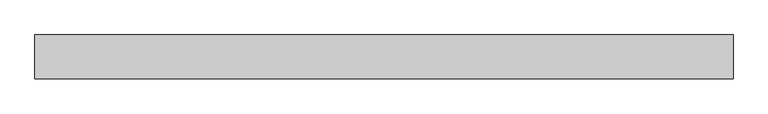
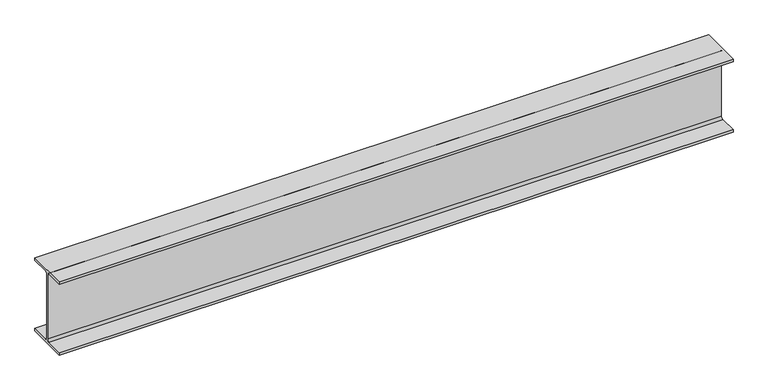
"""IFC4 building model written with IfcOpenShell, lengths in millimetres: beam geometry, Steel Beam_H-KSD3502 : H_SB_ASB_H-250x125x6x9."""

import ifcopenshell
import ifcopenshell.guid

model = None  # the IFC model being written
_history = None  # IfcOwnerHistory: only IFC2X3 demands one
_inside = {}  # id of a spatial element -> (the spatial element, [elements in it])
_under = {}  # id of a project, library or spatial element -> (it, [spatial elements below it])
_declared = {}  # id of a project -> (the project, [libraries it declares])
_typed = {}  # id of a type object -> (the type object, [elements of that type])
_made_of = {}  # id of a material, layer set ... -> (it, [elements and type objects made of it])


def new_model(schema):
    """Start an empty IFC model of exactly this schema.

    Asked for "IFC4X3", IfcOpenShell would pick the latest addendum, in which some entities
    have other attributes; the version numbers below select the first issue.
    IFC2X3 requires an IfcOwnerHistory on every rooted entity: one is made here for all.
    """
    global model, _history
    if schema == "IFC4X3":
        model = ifcopenshell.file(schema_version=(4, 3, 0, 0))
    else:
        model = ifcopenshell.file(schema=schema)
    _inside.clear()
    _under.clear()
    _declared.clear()
    _typed.clear()
    _made_of.clear()
    _history = None
    if model.schema == "IFC2X3":
        org = make("IfcOrganization", Name="unknown")
        user = make(
            "IfcPersonAndOrganization",
            ThePerson=make("IfcPerson", FamilyName="unknown"),
            TheOrganization=org,
        )
        app = make(
            "IfcApplication",
            ApplicationDeveloper=org,
            Version="unknown",
            ApplicationFullName="unknown",
            ApplicationIdentifier="unknown",
        )
        _history = make(
            "IfcOwnerHistory",
            OwningUser=user,
            OwningApplication=app,
            ChangeAction="ADDED",
            CreationDate=0,
        )
    return model


def make(cls, **values):
    """One entity of the class cls with the attributes given. An attribute that is None is left unset."""
    return model.create_entity(
        cls, **{name: value for name, value in values.items() if value is not None}
    )


def rooted(cls, **values):
    """An entity with a GlobalId (a new one), such as an element, a storey or a relation."""
    return make(cls, GlobalId=ifcopenshell.guid.new(), OwnerHistory=_history, **values)


def si_unit(unit_type, name, prefix=None):
    """IfcSIUnit, for example si_unit("LENGTHUNIT", "METRE", prefix="MILLI")."""
    return make("IfcSIUnit", UnitType=unit_type, Prefix=prefix, Name=name)


def assignment(units):
    """IfcUnitAssignment: the units of a project."""
    return None if units is None else make("IfcUnitAssignment", Units=units)


def point(xyz):
    """IfcCartesianPoint."""
    return None if xyz is None else make("IfcCartesianPoint", Coordinates=xyz)


def direction(xyz):
    """IfcDirection."""
    return None if xyz is None else make("IfcDirection", DirectionRatios=xyz)


def frame(location, z_axis=None, x_axis=None):
    """IfcAxis2Placement3D, a coordinate frame: its origin and axes. An axis left out is left unset."""
    return make(
        "IfcAxis2Placement3D",
        Location=point(location),
        Axis=direction(z_axis),
        RefDirection=direction(x_axis),
    )


def frame_2d(location, x_axis=None):
    """IfcAxis2Placement2D, a coordinate frame in the plane: its origin and x axis."""
    return make(
        "IfcAxis2Placement2D", Location=point(location), RefDirection=direction(x_axis)
    )


def origin():
    """The frame at (0, 0, 0) with its axes left unset."""
    return frame((0.0, 0.0, 0.0))


def place(relative_to, where):
    """IfcLocalPlacement: puts the frame where relative to a parent placement (None: the world)."""
    return make(
        "IfcLocalPlacement", PlacementRelTo=relative_to, RelativePlacement=where
    )


def context(
    kind, dimensions, precision=None, world=None, true_north=None, identifier=None
):
    """IfcGeometricRepresentationContext, for example the 3D "Model" context."""
    return make(
        "IfcGeometricRepresentationContext",
        ContextIdentifier=identifier,
        ContextType=kind,
        CoordinateSpaceDimension=dimensions,
        Precision=precision,
        WorldCoordinateSystem=world,
        TrueNorth=true_north,
    )


def project(units=None, contexts=None):
    """IfcProject with its units and contexts."""
    return rooted(
        "IfcProject",
        Name="project",
        RepresentationContexts=contexts,
        UnitsInContext=assignment(units),
    )


def spatial(cls, under=None, at=None, **own):
    """A site, building, storey or space (cls), placed at a placement, below another one or the project."""
    s = rooted(cls, ObjectPlacement=at, **own)
    if under is not None:
        _under.setdefault(under.id(), (under, []))[1].append(s)
    return s


def polyline(points):
    """IfcPolyline through the points."""
    return make("IfcPolyline", Points=[point(p) for p in points])


def circle_curve(where, radius):
    """IfcCircle in the frame where."""
    return make("IfcCircle", Position=where, Radius=radius)


def trimmed(basis, trim1, trim2, sense, master):
    """IfcTrimmedCurve: the piece of a basis curve between two trims."""
    return make(
        "IfcTrimmedCurve",
        BasisCurve=basis,
        Trim1=trim1,
        Trim2=trim2,
        SenseAgreement=sense,
        MasterRepresentation=master,
    )


def segment(curve, same_sense, transition):
    """IfcCompositeCurveSegment."""
    return make(
        "IfcCompositeCurveSegment",
        Transition=transition,
        SameSense=same_sense,
        ParentCurve=curve,
    )


def composite_curve(segments, self_intersect=None):
    """IfcCompositeCurve: segments joined end to end."""
    return make("IfcCompositeCurve", Segments=segments, SelfIntersect=self_intersect)


def outline(outer, holes=None, kind="AREA"):
    """IfcArbitraryClosedProfileDef: a profile drawn as a closed curve; with holes, ...WithVoids."""
    if holes is None:
        return make("IfcArbitraryClosedProfileDef", ProfileType=kind, OuterCurve=outer)
    return make(
        "IfcArbitraryProfileDefWithVoids",
        ProfileType=kind,
        OuterCurve=outer,
        InnerCurves=holes,
    )


def extrude(swept, where, along, depth):
    """IfcExtrudedAreaSolid: the profile swept, set in the frame where, extruded along a direction by depth."""
    return make(
        "IfcExtrudedAreaSolid",
        SweptArea=swept,
        Position=where,
        ExtrudedDirection=direction(along),
        Depth=depth,
    )


def shape(context_of_items, identifier, shape_type, items):
    """IfcShapeRepresentation: the items that make up one representation, for example the "Body"."""
    return make(
        "IfcShapeRepresentation",
        ContextOfItems=context_of_items,
        RepresentationIdentifier=identifier,
        RepresentationType=shape_type,
        Items=items,
    )


def source(mapping_origin, context_of_items, identifier, shape_type, items):
    """IfcRepresentationMap: a shape defined once, which mapped items show again and again."""
    return make(
        "IfcRepresentationMap",
        MappingOrigin=mapping_origin,
        MappedRepresentation=shape(context_of_items, identifier, shape_type, items),
    )


def transform(
    local_origin,
    x_axis=None,
    y_axis=None,
    z_axis=None,
    scale=None,
    scale2=None,
    scale3=None,
    uniform=True,
):
    """IfcCartesianTransformationOperator3D, or its non-uniform kind. x_axis, y_axis, z_axis: its Axis1, 2, 3."""
    if uniform:
        return make(
            "IfcCartesianTransformationOperator3D",
            Axis1=direction(x_axis),
            Axis2=direction(y_axis),
            LocalOrigin=point(local_origin),
            Scale=scale,
            Axis3=direction(z_axis),
        )
    return make(
        "IfcCartesianTransformationOperator3DnonUniform",
        Axis1=direction(x_axis),
        Axis2=direction(y_axis),
        LocalOrigin=point(local_origin),
        Scale=scale,
        Axis3=direction(z_axis),
        Scale2=scale2,
        Scale3=scale3,
    )


def mapped(mapping_source, mapping_target):
    """IfcMappedItem: shows the shape of a source again, moved by a transform."""
    return make(
        "IfcMappedItem", MappingSource=mapping_source, MappingTarget=mapping_target
    )


def made_of(thing, what):
    """Note that an element or type object is made of a material, layer set ...; save() writes the relation."""
    if what is not None:
        _made_of.setdefault(what.id(), (what, []))[1].append(thing)
    return thing


def element(
    cls,
    number,
    at=None,
    inside=None,
    cuts=None,
    type_object=None,
    material=None,
    context=None,
    identifier="Body",
    shape_type=None,
    held_by="IfcProductDefinitionShape",
    body=None,
    shapes=None,
    **own,
):
    """One element of the class cls, such as IfcWall. Its Tag is "e" and its number.

    at: its placement. inside: the storey or other place that contains it. cuts: it is an
    opening in that element (IfcRelVoidsElement). A single representation is given by context,
    identifier, shape_type and body (its items); several are given by shapes. held_by: the class
    of the entity that holds the representations. save() writes the other relations.
    """
    e = rooted(cls, Tag="e%d" % number, ObjectPlacement=at, **own)
    if body is not None:
        shapes = [shape(context, identifier, shape_type, body)]
    if shapes is not None:
        e.Representation = make(held_by, Representations=shapes)
    if inside is not None:
        _inside.setdefault(inside.id(), (inside, []))[1].append(e)
    if cuts is not None:
        rooted(
            "IfcRelVoidsElement", RelatingBuildingElement=cuts, RelatedOpeningElement=e
        )
    if type_object is not None:
        _typed.setdefault(type_object.id(), (type_object, []))[1].append(e)
    return made_of(e, material)


def aggregate(whole, parts):
    """IfcRelAggregates: a whole, such as a stair, and the parts it consists of."""
    return rooted("IfcRelAggregates", RelatingObject=whole, RelatedObjects=parts)


def save(model, path):
    """Write the relations noted so far, then the file.

    IfcRelAggregates (storeys below a building ...), IfcRelContainedInSpatialStructure (elements
    in a storey), IfcRelDefinesByType, IfcRelAssociatesMaterial and IfcRelDeclares: one each for
    every whole, place, type object, material and project.
    """
    for whole, parts in _under.values():
        aggregate(whole, parts)
    for where, things in _inside.values():
        rooted(
            "IfcRelContainedInSpatialStructure",
            RelatedElements=things,
            RelatingStructure=where,
        )
    for kind, things in _typed.values():
        rooted("IfcRelDefinesByType", RelatedObjects=things, RelatingType=kind)
    for what, things in _made_of.values():
        rooted("IfcRelAssociatesMaterial", RelatedObjects=things, RelatingMaterial=what)
    for by, libraries in _declared.values():
        rooted("IfcRelDeclares", RelatingContext=by, RelatedDefinitions=libraries)
    model.write(path)


def beam_b5d638d0(model_context):
    return source(origin(), model_context, "Body", "SweptSolid", [
        extrude(outline(composite_curve([segment(polyline([(82.5, -141.5), (82.5, -151.7), (-82.5, -151.7), (-82.5, -141.5), (-11.9, -141.5)]), True, "CONTINUOUS"), segment(trimmed(circle_curve(frame_2d((-11.9, -132.6)), 8.9), [point((-11.9, -141.5))], [point((-3.0, -132.6))], True, "CARTESIAN"), True, "CONTINUOUS"), segment(polyline([(-3.0, -132.6), (-3.0, 132.6)]), True, "CONTINUOUS"), segment(trimmed(circle_curve(frame_2d((-11.9, 132.6)), 8.9), [point((-3.0, 132.6))], [point((-11.9, 141.5))], True, "CARTESIAN"), True, "CONTINUOUS"), segment(polyline([(-11.9, 141.5), (-82.5, 141.5), (-82.5, 151.7), (82.5, 151.7), (82.5, 141.5), (11.9, 141.5)]), True, "CONTINUOUS"), segment(trimmed(circle_curve(frame_2d((11.9, 132.6)), 8.9), [point((11.9, 141.5))], [point((3.0, 132.6))], True, "CARTESIAN"), True, "CONTINUOUS"), segment(polyline([(3.0, 132.6), (3.0, -132.6)]), True, "CONTINUOUS"), segment(trimmed(circle_curve(frame_2d((11.9, -132.6)), 8.9), [point((3.0, -132.6))], [point((11.9, -141.5))], True, "CARTESIAN"), True, "CONTINUOUS"), segment(polyline([(11.9, -141.5), (82.5, -141.5)]), True, "CONTINUOUS")], self_intersect=False)), frame((-1387.3, 0.0, 0.0), z_axis=(1.0, 0.0, 0.0), x_axis=(0.0, 1.0, 0.0)), (0.0, 0.0, 1.0), 2636.6),
    ])


if __name__ == "__main__":
    model = new_model("IFC4")
    model_context = context("Model", 3, world=origin())
    ifc_project = project(units=[si_unit("LENGTHUNIT", "METRE", prefix="MILLI")], contexts=[model_context])
    site = spatial("IfcSite", under=ifc_project)
    building = spatial("IfcBuilding", under=site)
    placement = place(None, origin())
    beam_shape = beam_b5d638d0(model_context)
    element("IfcBeam", 1, ObjectType="Steel Beam_H-KSD3502 : H_SB_ASB_H-250x125x6x9", at=placement, inside=building, context=model_context, shape_type="MappedRepresentation", body=[
        mapped(beam_shape, transform((0.0, 0.0, 0.0), x_axis=(1.0, 0.0, 0.0), y_axis=(0.0, 1.0, 0.0), z_axis=(0.0, 0.0, 1.0))),
    ])
    save(model, "model.ifc")

# Revit data of these elements
# Type "Steel Beam_H-KSD3502 : H_SB_ASB_H-250x125x6x9"
#   Width = 12.5 cm
#   Web Thickness = 0.6 cm
#   Web Fillet = 1.2 cm
#   Warping Constant = 42539.8 cm⁶
#   Torsional Moment of Inertia = 7.8102 cm⁴
#   Torsional Modulus = 1.0 cm³
#   Section Area = 37.66 cm²
#   Plastic Modulus weak axis = 73.1 cm³
#   Plastic Modulus strong axis = 366.0 cm³
#   Perimeter = 0.97 m²/m
#   Nominal Weight = 29.60 kgf/m
#   Moment of Inertia weak axis = 294.00 cm⁴
#   Moment of Inertia strong axis = 4050.00 cm⁴
#   Height = 25.0 cm
#   Flange Thickness = 0.9 cm
#   Elastic Modulus weak axis = 47.0 cm³
#   Elastic Modulus strong axis = 324.0 cm³
#   Centroid Vertical = 12.5 cm
#   Centroid Horizontal = 6.25 cm
#   Length [instance default] = 1.5240 m
#   Structural Material [instance default] = Steel, 45-345
#   Assembly Code = ""
# Element 1 (IfcBeam, "Steel Beam_H-KSD3502 : H_SB_ASB_H-250x125x6x9")
#   Structural Material = none
# Materials
#   "Steel, 45-345": class "Metal", colour RGB 189 187 185, transparency 0, Description = "Steel 345 MPa", Cost = 0
